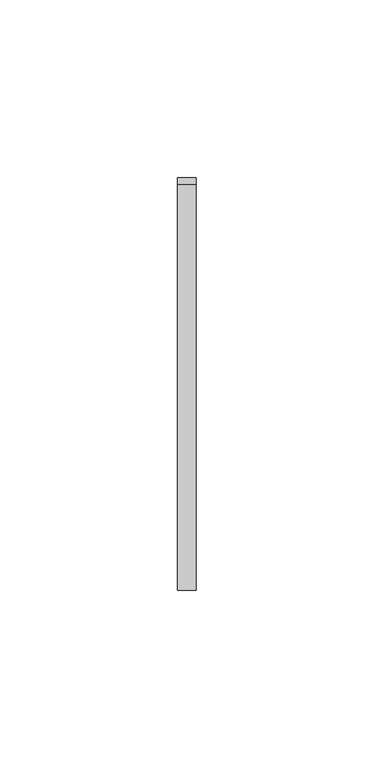
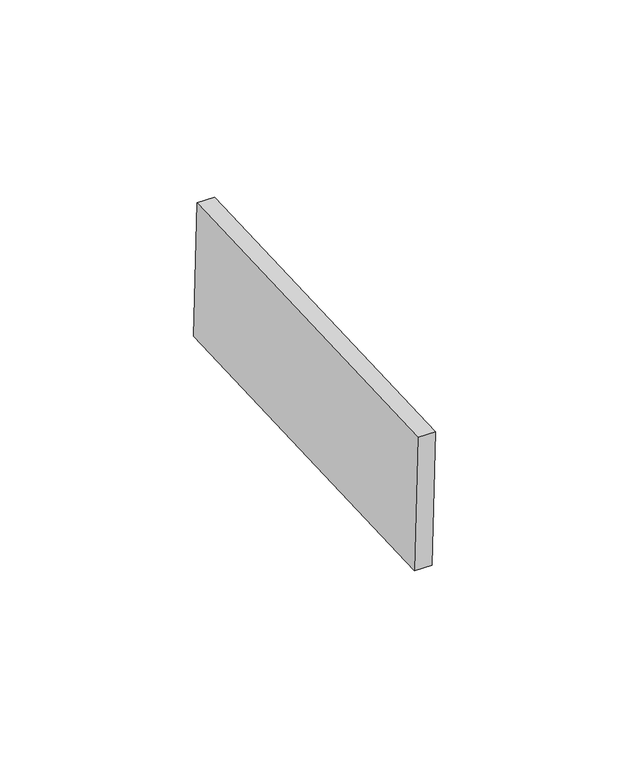
"""IFC4 building model written with IfcOpenShell, lengths in millimetres: proxy geometry, Inner panel:Inner panel:1:Inner panel:1 : Inner panel:Inner panel:300324:2:Inner panel:1:Inner panel:1 : Inner panel:Inner panel:300324:2 : Inner panel:Inner panel:1:Inner panel:1 : Inner panel:Inner panel:300324:300043:50 : Inner panel:Inner panel:1:Inner panel:1 : Inner panel:Inner panel:300324:2:Inner panel:1:Inner panel:1 : Inner panel:Inner panel:300324:2 : Inner panel:Inner panel:1:Inner panel:1 : Inner panel:Inner panel:300324:300043:308120."""

import ifcopenshell
import ifcopenshell.guid

model = None  # the IFC model being written
_history = None  # IfcOwnerHistory: only IFC2X3 demands one
_inside = {}  # id of a spatial element -> (the spatial element, [elements in it])
_under = {}  # id of a project, library or spatial element -> (it, [spatial elements below it])
_declared = {}  # id of a project -> (the project, [libraries it declares])
_typed = {}  # id of a type object -> (the type object, [elements of that type])
_made_of = {}  # id of a material, layer set ... -> (it, [elements and type objects made of it])


def new_model(schema):
    """Start an empty IFC model of exactly this schema.

    Asked for "IFC4X3", IfcOpenShell would pick the latest addendum, in which some entities
    have other attributes; the version numbers below select the first issue.
    IFC2X3 requires an IfcOwnerHistory on every rooted entity: one is made here for all.
    """
    global model, _history
    if schema == "IFC4X3":
        model = ifcopenshell.file(schema_version=(4, 3, 0, 0))
    else:
        model = ifcopenshell.file(schema=schema)
    _inside.clear()
    _under.clear()
    _declared.clear()
    _typed.clear()
    _made_of.clear()
    _history = None
    if model.schema == "IFC2X3":
        org = make("IfcOrganization", Name="unknown")
        user = make(
            "IfcPersonAndOrganization",
            ThePerson=make("IfcPerson", FamilyName="unknown"),
            TheOrganization=org,
        )
        app = make(
            "IfcApplication",
            ApplicationDeveloper=org,
            Version="unknown",
            ApplicationFullName="unknown",
            ApplicationIdentifier="unknown",
        )
        _history = make(
            "IfcOwnerHistory",
            OwningUser=user,
            OwningApplication=app,
            ChangeAction="ADDED",
            CreationDate=0,
        )
    return model


def make(cls, **values):
    """One entity of the class cls with the attributes given. An attribute that is None is left unset."""
    return model.create_entity(
        cls, **{name: value for name, value in values.items() if value is not None}
    )


def rooted(cls, **values):
    """An entity with a GlobalId (a new one), such as an element, a storey or a relation."""
    return make(cls, GlobalId=ifcopenshell.guid.new(), OwnerHistory=_history, **values)


def si_unit(unit_type, name, prefix=None):
    """IfcSIUnit, for example si_unit("LENGTHUNIT", "METRE", prefix="MILLI")."""
    return make("IfcSIUnit", UnitType=unit_type, Prefix=prefix, Name=name)


def assignment(units):
    """IfcUnitAssignment: the units of a project."""
    return None if units is None else make("IfcUnitAssignment", Units=units)


def point(xyz):
    """IfcCartesianPoint."""
    return None if xyz is None else make("IfcCartesianPoint", Coordinates=xyz)


def direction(xyz):
    """IfcDirection."""
    return None if xyz is None else make("IfcDirection", DirectionRatios=xyz)


def frame(location, z_axis=None, x_axis=None):
    """IfcAxis2Placement3D, a coordinate frame: its origin and axes. An axis left out is left unset."""
    return make(
        "IfcAxis2Placement3D",
        Location=point(location),
        Axis=direction(z_axis),
        RefDirection=direction(x_axis),
    )


def origin():
    """The frame at (0, 0, 0) with its axes left unset."""
    return frame((0.0, 0.0, 0.0))


def place(relative_to, where):
    """IfcLocalPlacement: puts the frame where relative to a parent placement (None: the world)."""
    return make(
        "IfcLocalPlacement", PlacementRelTo=relative_to, RelativePlacement=where
    )


def context(
    kind, dimensions, precision=None, world=None, true_north=None, identifier=None
):
    """IfcGeometricRepresentationContext, for example the 3D "Model" context."""
    return make(
        "IfcGeometricRepresentationContext",
        ContextIdentifier=identifier,
        ContextType=kind,
        CoordinateSpaceDimension=dimensions,
        Precision=precision,
        WorldCoordinateSystem=world,
        TrueNorth=true_north,
    )


def project(units=None, contexts=None):
    """IfcProject with its units and contexts."""
    return rooted(
        "IfcProject",
        Name="project",
        RepresentationContexts=contexts,
        UnitsInContext=assignment(units),
    )


def spatial(cls, under=None, at=None, **own):
    """A site, building, storey or space (cls), placed at a placement, below another one or the project."""
    s = rooted(cls, ObjectPlacement=at, **own)
    if under is not None:
        _under.setdefault(under.id(), (under, []))[1].append(s)
    return s


def polyline(points):
    """IfcPolyline through the points."""
    return make("IfcPolyline", Points=[point(p) for p in points])


def outline(outer, holes=None, kind="AREA"):
    """IfcArbitraryClosedProfileDef: a profile drawn as a closed curve; with holes, ...WithVoids."""
    if holes is None:
        return make("IfcArbitraryClosedProfileDef", ProfileType=kind, OuterCurve=outer)
    return make(
        "IfcArbitraryProfileDefWithVoids",
        ProfileType=kind,
        OuterCurve=outer,
        InnerCurves=holes,
    )


def extrude(swept, where, along, depth):
    """IfcExtrudedAreaSolid: the profile swept, set in the frame where, extruded along a direction by depth."""
    return make(
        "IfcExtrudedAreaSolid",
        SweptArea=swept,
        Position=where,
        ExtrudedDirection=direction(along),
        Depth=depth,
    )


def shape(context_of_items, identifier, shape_type, items):
    """IfcShapeRepresentation: the items that make up one representation, for example the "Body"."""
    return make(
        "IfcShapeRepresentation",
        ContextOfItems=context_of_items,
        RepresentationIdentifier=identifier,
        RepresentationType=shape_type,
        Items=items,
    )


def source(mapping_origin, context_of_items, identifier, shape_type, items):
    """IfcRepresentationMap: a shape defined once, which mapped items show again and again."""
    return make(
        "IfcRepresentationMap",
        MappingOrigin=mapping_origin,
        MappedRepresentation=shape(context_of_items, identifier, shape_type, items),
    )


def transform(
    local_origin,
    x_axis=None,
    y_axis=None,
    z_axis=None,
    scale=None,
    scale2=None,
    scale3=None,
    uniform=True,
):
    """IfcCartesianTransformationOperator3D, or its non-uniform kind. x_axis, y_axis, z_axis: its Axis1, 2, 3."""
    if uniform:
        return make(
            "IfcCartesianTransformationOperator3D",
            Axis1=direction(x_axis),
            Axis2=direction(y_axis),
            LocalOrigin=point(local_origin),
            Scale=scale,
            Axis3=direction(z_axis),
        )
    return make(
        "IfcCartesianTransformationOperator3DnonUniform",
        Axis1=direction(x_axis),
        Axis2=direction(y_axis),
        LocalOrigin=point(local_origin),
        Scale=scale,
        Axis3=direction(z_axis),
        Scale2=scale2,
        Scale3=scale3,
    )


def mapped(mapping_source, mapping_target):
    """IfcMappedItem: shows the shape of a source again, moved by a transform."""
    return make(
        "IfcMappedItem", MappingSource=mapping_source, MappingTarget=mapping_target
    )


def made_of(thing, what):
    """Note that an element or type object is made of a material, layer set ...; save() writes the relation."""
    if what is not None:
        _made_of.setdefault(what.id(), (what, []))[1].append(thing)
    return thing


def element(
    cls,
    number,
    at=None,
    inside=None,
    cuts=None,
    type_object=None,
    material=None,
    context=None,
    identifier="Body",
    shape_type=None,
    held_by="IfcProductDefinitionShape",
    body=None,
    shapes=None,
    **own,
):
    """One element of the class cls, such as IfcWall. Its Tag is "e" and its number.

    at: its placement. inside: the storey or other place that contains it. cuts: it is an
    opening in that element (IfcRelVoidsElement). A single representation is given by context,
    identifier, shape_type and body (its items); several are given by shapes. held_by: the class
    of the entity that holds the representations. save() writes the other relations.
    """
    e = rooted(cls, Tag="e%d" % number, ObjectPlacement=at, **own)
    if body is not None:
        shapes = [shape(context, identifier, shape_type, body)]
    if shapes is not None:
        e.Representation = make(held_by, Representations=shapes)
    if inside is not None:
        _inside.setdefault(inside.id(), (inside, []))[1].append(e)
    if cuts is not None:
        rooted(
            "IfcRelVoidsElement", RelatingBuildingElement=cuts, RelatedOpeningElement=e
        )
    if type_object is not None:
        _typed.setdefault(type_object.id(), (type_object, []))[1].append(e)
    return made_of(e, material)


def aggregate(whole, parts):
    """IfcRelAggregates: a whole, such as a stair, and the parts it consists of."""
    return rooted("IfcRelAggregates", RelatingObject=whole, RelatedObjects=parts)


def save(model, path):
    """Write the relations noted so far, then the file.

    IfcRelAggregates (storeys below a building ...), IfcRelContainedInSpatialStructure (elements
    in a storey), IfcRelDefinesByType, IfcRelAssociatesMaterial and IfcRelDeclares: one each for
    every whole, place, type object, material and project.
    """
    for whole, parts in _under.values():
        aggregate(whole, parts)
    for where, things in _inside.values():
        rooted(
            "IfcRelContainedInSpatialStructure",
            RelatedElements=things,
            RelatingStructure=where,
        )
    for kind, things in _typed.values():
        rooted("IfcRelDefinesByType", RelatedObjects=things, RelatingType=kind)
    for what, things in _made_of.values():
        rooted("IfcRelAssociatesMaterial", RelatedObjects=things, RelatingMaterial=what)
    for by, libraries in _declared.values():
        rooted("IfcRelDeclares", RelatingContext=by, RelatedDefinitions=libraries)
    model.write(path)


def generic_models_1a555196(model_context):
    return source(origin(), model_context, "Body", "SweptSolid", [
        extrude(outline(polyline([(0.0, -114.2999999), (0.0, 0.0), (5.2138089, 0.0), (5.2138089, -114.2999999), (0.0, -114.2999999)])), frame((593530.195117, -566950.1308393, 8857.6957503), z_axis=(0.0, -0.04163054471215927, 0.9991330730923529), x_axis=(-1.0, 0.0, 0.0)), (0.0, 0.0, 1.0), 43.2233908),
    ])


if __name__ == "__main__":
    model = new_model("IFC4")
    model_context = context("Model", 3, world=origin())
    ifc_project = project(units=[si_unit("LENGTHUNIT", "METRE", prefix="MILLI")], contexts=[model_context])
    site = spatial("IfcSite", under=ifc_project)
    building = spatial("IfcBuilding", under=site)
    placement = place(None, origin())
    generic_models_shape = generic_models_1a555196(model_context)
    element("IfcBuildingElementProxy", 1, Name="Inner panel:Inner panel:1:Inner panel:1 : Inner panel:Inner panel:300324:2:Inner panel:1:Inner panel:1 : Inner panel:Inner panel:300324:2 : Inner panel:Inner panel:1:Inner panel:1 : Inner panel:Inner panel:300324:300043:50 : Inner panel:Inner panel:1:Inner panel:1 : Inner panel:Inner panel:300324:2:Inner panel:1:Inner panel:1 : Inner panel:Inner panel:300324:2 : Inner panel:Inner panel:1:Inner panel:1 : Inner panel:Inner panel:300324:300043:308120", ObjectType="Inner panel:Inner panel:1:Inner panel:1 : Inner panel:Inner panel:300324:2:Inner panel:1:Inner panel:1 : Inner panel:Inner panel:300324:2 : Inner panel:Inner panel:1:Inner panel:1 : Inner panel:Inner panel:300324:300043:50 : Inner panel:Inner panel:1:Inner panel:1 : Inner panel:Inner panel:300324:2:Inner panel:1:Inner panel:1 : Inner panel:Inner panel:300324:2 : Inner panel:Inner panel:1:Inner panel:1 : Inner panel:Inner panel:300324:300043:308120", at=placement, inside=building, context=model_context, shape_type="MappedRepresentation", body=[
        mapped(generic_models_shape, transform((0.0, 0.0, 0.0), x_axis=(1.0, 0.0, 0.0), y_axis=(0.0, 1.0, 0.0), z_axis=(0.0, 0.0, 1.0))),
    ])
    save(model, "model.ifc")

# Revit data of these elements
# Type "Inner panel:Inner panel:1:Inner panel:1 : Inner panel:Inner panel:300324:2:Inner panel:1:Inner panel:1 : Inner panel:Inner panel:300324:2 : Inner panel:Inner panel:1:Inner panel:1 : Inner panel:Inner panel:300324:300043:50 : Inner panel:Inner panel:1:Inner panel:1 : Inner panel:Inner panel:300324:2:Inner panel:1:Inner panel:1 : Inner panel:Inner panel:300324:2 : Inner panel:Inner panel:1:Inner panel:1 : Inner panel:Inner panel:300324:300043:308120"
#   NameOverride = "Inner panel:Inner panel:1:Inner panel:1 : Inner panel:Inner panel:300324:2:Inner panel:1:Inner panel:1 : Inner panel:Inner panel:300324:2 : Inner panel:Inner panel:1:Inner panel:1 : Inner panel:Inner panel:300324:300043:308120"
#   ObjectTypeOverride = "Inner panel:1:Inner panel:1 : Inner panel:Inner panel:300324:2 : Inner panel:Inner panel:1:Inner panel:1 : Inner panel:Inner panel:300324:300043"
#   Reference = "Inner panel"
#   Tag = "308120"
# Element 1 (IfcBuildingElementProxy, "Inner panel:Inner panel:1:Inner panel:1 : Inner panel:Inner panel:300324:2:Inner panel:1:Inner panel:1 : Inner panel:Inner panel:300324:2 : Inner panel:Inner panel:1:Inner panel:1 : Inner panel:Inner panel:300324:300043:50 : Inner panel:Inner panel:1:Inner panel:1 : Inner panel:Inner panel:300324:2:Inner panel:1:Inner panel:1 : Inner panel:Inner panel:300324:2 : Inner panel:Inner panel:1:Inner panel:1 : Inner panel:Inner panel:300324:300043:308120")
#   Materials on its faces: "SLIDING CLIP"
# Materials
#   "SLIDING CLIP": class "Generic", colour RGB 120 120 120, transparency 0, Cost = 0
